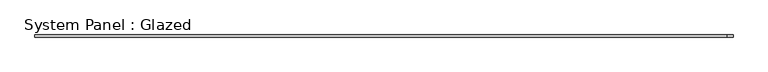
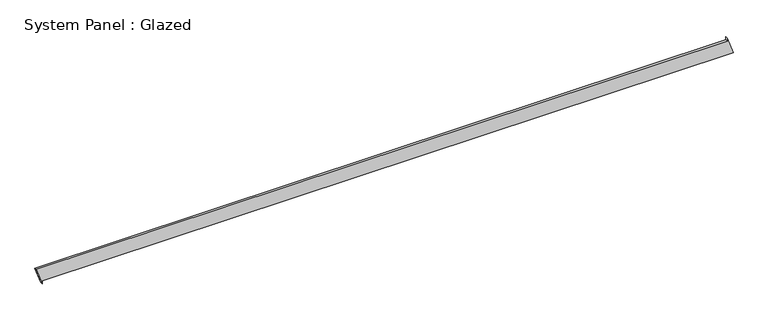
"""IFC4 building model written with IfcOpenShell, lengths in millimetres: plate geometry, System Panel : Glazed."""

from ifc_helpers import new_model, si_unit, frame, origin, place, context, project, spatial, polyline, outline, extrude, source, transform, mapped, element, save


def system_panel_glazed_1d5d9c82(model_context):
    return source(origin(), model_context, "Body", "SweptSolid", [
        extrude(outline(polyline([(0.0, -3957.7762608), (35.3553391, -3957.7762608), (35.3553391, 4027.3165452), (235.5515472, 3958.146555), (200.1962081, 3958.1472368), (200.0422004, -4027.3165452), (0.0, -3957.7762608)])), frame((0.0, -49.5, 0.0), z_axis=(0.0, 1.0, 0.0), x_axis=(0.0, 0.0, 1.0)), (0.0, 0.0, 1.0), 25.0),
    ])


if __name__ == "__main__":
    model = new_model("IFC4")
    model_context = context("Model", 3, world=origin())
    ifc_project = project(units=[si_unit("LENGTHUNIT", "METRE", prefix="MILLI")], contexts=[model_context])
    site = spatial("IfcSite", under=ifc_project)
    building = spatial("IfcBuilding", under=site)
    placement = place(None, origin())
    system_panel_glazed_shape = system_panel_glazed_1d5d9c82(model_context)
    element("IfcPlate", 1, ObjectType="System Panel : Glazed", at=placement, inside=building, context=model_context, shape_type="MappedRepresentation", body=[
        mapped(system_panel_glazed_shape, transform((0.0, 0.0, 0.0), x_axis=(1.0, 0.0, 0.0), y_axis=(0.0, 1.0, 0.0), z_axis=(0.0, 0.0, 1.0))),
    ])
    save(model, "model.ifc")

# Revit data of these elements
# Element 1 (IfcPlate, "System Panel : Glazed")
#   Materials on its faces: "Glass"
# Materials
#   "Glass": class "Glass", colour RGB 218 227 224, transparency 0.85, Description = "Soda Lime Glass", Cost = 0
